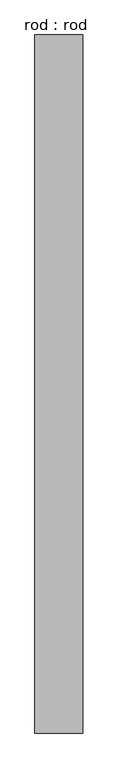
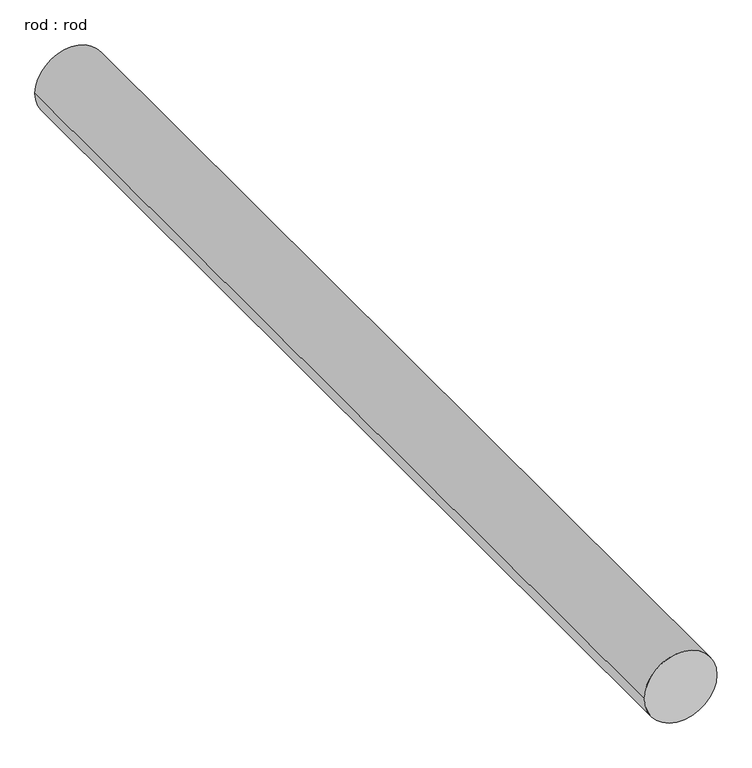
"""IFC4 building model written with IfcOpenShell, lengths in millimetres: proxy geometry, rod : rod."""

from ifc_helpers import new_model, si_unit, point, frame, frame_2d, origin, place, context, project, spatial, circle_curve, trimmed, segment, composite_curve, outline, extrude, source, transform, mapped, element, save


def rod_rod_debf6b8e(model_context):
    return source(origin(), model_context, "Body", "SweptSolid", [
        extrude(outline(composite_curve([segment(trimmed(circle_curve(frame_2d((0.0108462, 0.0)), 200.0), [point((0.0108462, 200.0))], [point((0.0108462, -200.0))], False, "CARTESIAN"), True, "CONTINUOUS"), segment(trimmed(circle_curve(frame_2d((0.0108462, 0.0)), 200.0), [point((0.0108462, -200.0))], [point((0.0108462, 200.0))], False, "CARTESIAN"), True, "CONTINUOUS")], self_intersect=False)), frame((0.0, 1188.7070849, 0.0), z_axis=(0.0, 1.0, 0.0), x_axis=(0.0, 0.0, 1.0)), (0.0, 0.0, 1.0), 5808.0430609),
    ])


if __name__ == "__main__":
    model = new_model("IFC4")
    model_context = context("Model", 3, world=origin())
    ifc_project = project(units=[si_unit("LENGTHUNIT", "METRE", prefix="MILLI")], contexts=[model_context])
    site = spatial("IfcSite", under=ifc_project)
    building = spatial("IfcBuilding", under=site)
    placement = place(None, origin())
    rod_rod_shape = rod_rod_debf6b8e(model_context)
    element("IfcBuildingElementProxy", 1, Name="rod : rod", ObjectType="rod : rod", at=placement, inside=building, context=model_context, shape_type="MappedRepresentation", body=[
        mapped(rod_rod_shape, transform((0.0, 0.0, 0.0), x_axis=(1.0, 0.0, 0.0), y_axis=(0.0, 1.0, 0.0), z_axis=(0.0, 0.0, 1.0))),
    ])
    save(model, "model.ifc")

# Revit data of these elements
# Type "rod : rod"
#   Default Elevation = 0
